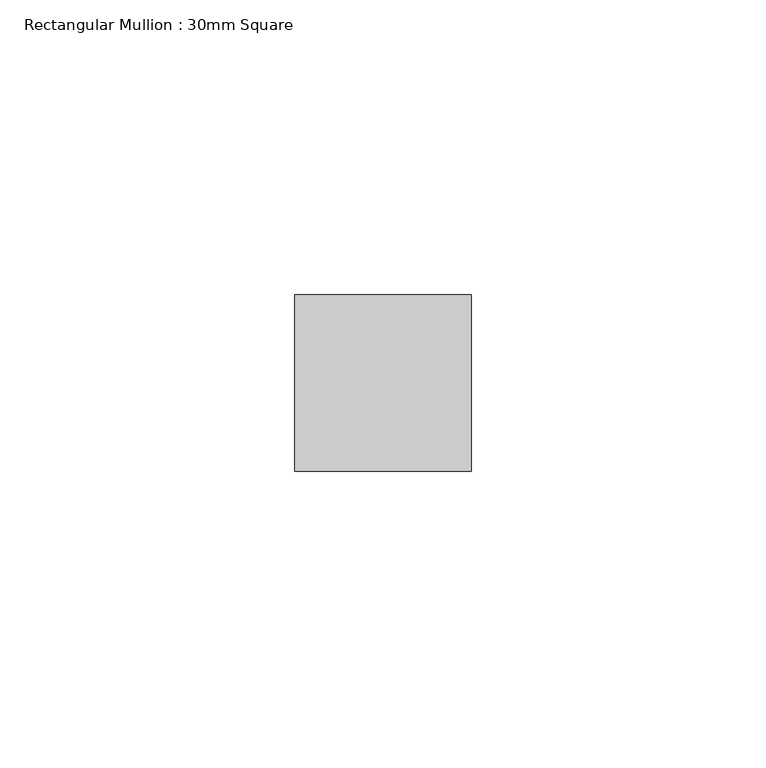
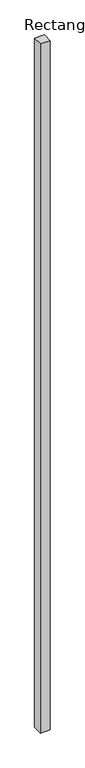
"""IFC4 building model written with IfcOpenShell, lengths in millimetres: member geometry, Rectangular Mullion : 30mm Square."""

from ifc_helpers import new_model, si_unit, frame, origin, place, context, project, spatial, polyline, outline, extrude, source, transform, mapped, element, save


def rectangular_mullion_30mm_square_f216c63b(model_context):
    return source(origin(), model_context, "Body", "SweptSolid", [
        extrude(outline(polyline([(15.0, 15.0), (15.0, -15.0), (-15.0, -15.0), (-15.0, 15.0), (15.0, 15.0)])), frame((0.0, 0.0, -2228.3891708), z_axis=(0.0, 0.0, 1.0), x_axis=(1.0, 0.0, 0.0)), (0.0, 0.0, 1.0), 2228.3891708),
    ])


if __name__ == "__main__":
    model = new_model("IFC4")
    model_context = context("Model", 3, world=origin())
    ifc_project = project(units=[si_unit("LENGTHUNIT", "METRE", prefix="MILLI")], contexts=[model_context])
    site = spatial("IfcSite", under=ifc_project)
    building = spatial("IfcBuilding", under=site)
    placement = place(None, origin())
    rectangular_mullion_30mm_square_shape = rectangular_mullion_30mm_square_f216c63b(model_context)
    element("IfcMember", 1, ObjectType="Rectangular Mullion : 30mm Square", at=placement, inside=building, context=model_context, shape_type="MappedRepresentation", body=[
        mapped(rectangular_mullion_30mm_square_shape, transform((0.0, 0.0, 0.0), x_axis=(1.0, 0.0, 0.0), y_axis=(0.0, 1.0, 0.0), z_axis=(0.0, 0.0, 1.0))),
    ])
    save(model, "model.ifc")

# Revit data of these elements
# Type "Rectangular Mullion : 30mm Square"
#   built-in parameter 1007304 = 0.0984252 (stored number, unit not read)
#   built-in parameter 1007301 = 0.0492126 (stored number, unit not read)
#   built-in parameter 1007300 = 0.0492126 (stored number, unit not read)
# Element 1 (IfcMember, "Rectangular Mullion : 30mm Square")
#   Materials on its faces: "Aluminum"
# Materials
#   "Aluminum": class "Metal", colour RGB 244 244 244, transparency 0, Description = "Aluminum 6061", Cost = 0
